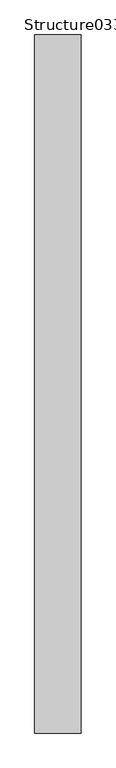
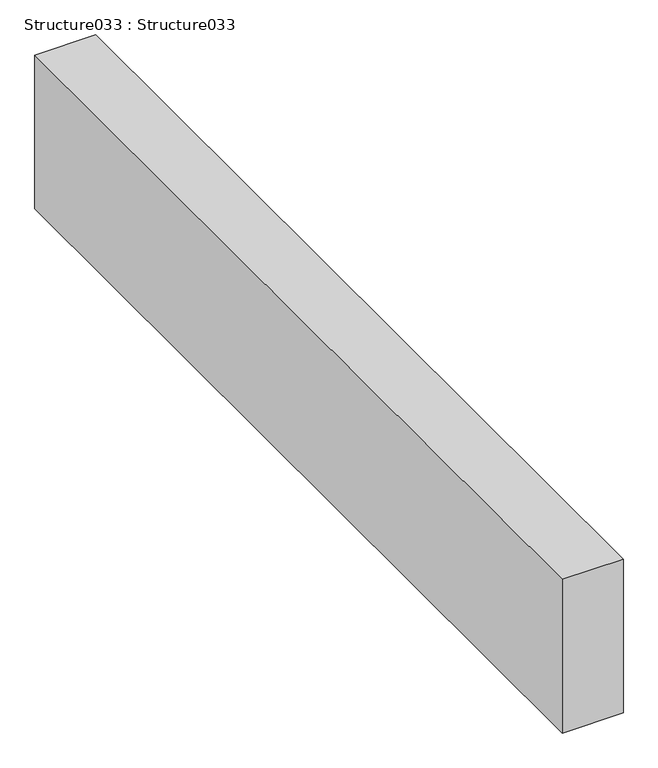
"""IFC4 building model written with IfcOpenShell, lengths in millimetres: proxy geometry, Structure033 : Structure033."""

from ifc_helpers import new_model, si_unit, frame, origin, place, context, project, spatial, polyline, outline, extrude, source, transform, mapped, element, save


def structure033_structure033_5b7dca5c(model_context):
    return source(origin(), model_context, "Body", "SweptSolid", [
        extrude(outline(polyline([(-6350.7711227, 7982.1531721), (-6484.1211227, 7982.1531721), (-6484.1211227, 9982.1531721), (-6350.7711227, 9982.1531721), (-6350.7711227, 7982.1531721)])), frame((0.0, 0.0, 43056.2082994), z_axis=(0.0, 0.0, 1.0), x_axis=(1.0, 0.0, 0.0)), (0.0, 0.0, 1.0), 355.6),
    ])


if __name__ == "__main__":
    model = new_model("IFC4")
    model_context = context("Model", 3, world=origin())
    ifc_project = project(units=[si_unit("LENGTHUNIT", "METRE", prefix="MILLI")], contexts=[model_context])
    site = spatial("IfcSite", under=ifc_project)
    building = spatial("IfcBuilding", under=site)
    placement = place(None, origin())
    structure033_structure033_shape = structure033_structure033_5b7dca5c(model_context)
    element("IfcBuildingElementProxy", 1, Name="Structure033 : Structure033", ObjectType="Structure033 : Structure033", at=placement, inside=building, context=model_context, shape_type="MappedRepresentation", body=[
        mapped(structure033_structure033_shape, transform((0.0, 0.0, 0.0), x_axis=(1.0, 0.0, 0.0), y_axis=(0.0, 1.0, 0.0), z_axis=(0.0, 0.0, 1.0))),
    ])
    save(model, "model.ifc")

# Revit data of these elements
# Type "Structure033 : Structure033"
#   NameOverride = "Structure033"
# Element 1 (IfcBuildingElementProxy, "Structure033 : Structure033")
#   Materials on its faces: "STRUCTURAL MEMBER (SEE STRUCTURAL DWGS)"
# Materials
#   "STRUCTURAL MEMBER (SEE STRUCTURAL DWGS)": class "Unassigned", colour RGB 176 134 95, transparency 0, Cost = 0
